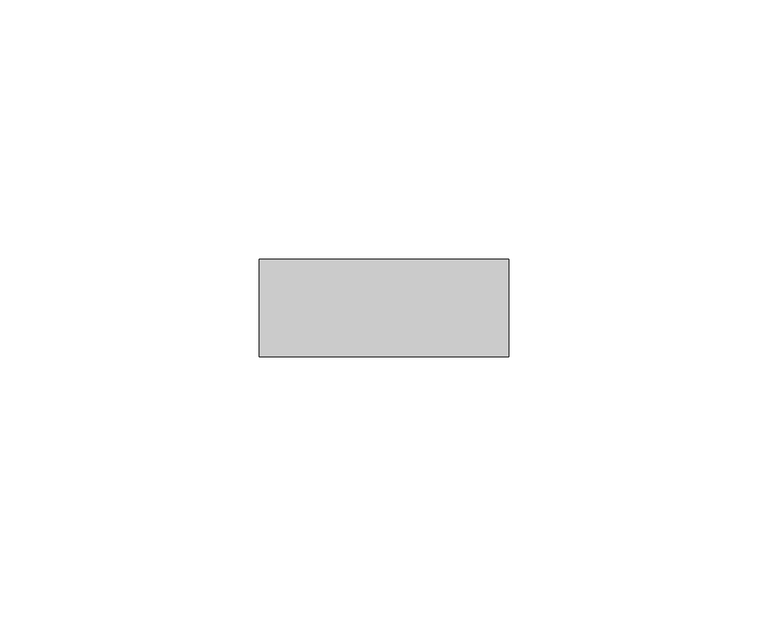
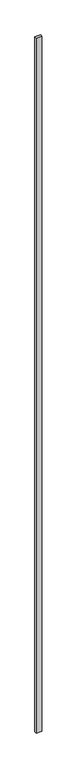
"""IFC4 building model written with IfcOpenShell, lengths in millimetres: proxy geometry, Generic Models 11:Generic Models 1:306267:Generic Models 1:306267 : Generic Models 11:Generic Models 1:306267:300405:Generic Models 1:306267:Generic Models 1:306267 : Generic Models 11:Generic Models 1:306267:300405 : Generic Models 11:Generic Models 1:306267:Generic Models 1:306267 : Generic Models 11:Generic Models 1:306267:300405:29 : Generic Models 11:Generic Models 1:306267:Generic Models 1:306267 : Generic Models 11:Generic Models 1:306267:300405:Generic Models 1:306267:Generic Models 1:306267 : Generic Models 11:Generic Models 1:306267:300405 : Generic Models 11:Generic Models 1:306267:Generic Models 1:306267 : Generic Models 11:Generic Models 1:306267:300405:300182."""

from ifc_helpers import new_model, si_unit, origin, origin_with_axes, place, context, project, spatial, polyline, outline, extrude, source, transform, mapped, element, save


def generic_models_2fd2b33c(model_context):
    return source(origin(), model_context, "Body", "SweptSolid", [
        extrude(outline(polyline([(667551.6493852, -568253.9540363), (667551.6493852, -568235.1560699), (667599.7284465, -568235.1560699), (667599.7284465, -568253.9540363), (667551.6493852, -568253.9540363)])), origin_with_axes(), (0.0, 0.0, 1.0), 6172.2),
    ])


if __name__ == "__main__":
    model = new_model("IFC4")
    model_context = context("Model", 3, world=origin())
    ifc_project = project(units=[si_unit("LENGTHUNIT", "METRE", prefix="MILLI")], contexts=[model_context])
    site = spatial("IfcSite", under=ifc_project)
    building = spatial("IfcBuilding", under=site)
    placement = place(None, origin())
    generic_models_shape = generic_models_2fd2b33c(model_context)
    element("IfcBuildingElementProxy", 1, Name="Generic Models 11:Generic Models 1:306267:Generic Models 1:306267 : Generic Models 11:Generic Models 1:306267:300405:Generic Models 1:306267:Generic Models 1:306267 : Generic Models 11:Generic Models 1:306267:300405 : Generic Models 11:Generic Models 1:306267:Generic Models 1:306267 : Generic Models 11:Generic Models 1:306267:300405:29 : Generic Models 11:Generic Models 1:306267:Generic Models 1:306267 : Generic Models 11:Generic Models 1:306267:300405:Generic Models 1:306267:Generic Models 1:306267 : Generic Models 11:Generic Models 1:306267:300405 : Generic Models 11:Generic Models 1:306267:Generic Models 1:306267 : Generic Models 11:Generic Models 1:306267:300405:300182", ObjectType="Generic Models 11:Generic Models 1:306267:Generic Models 1:306267 : Generic Models 11:Generic Models 1:306267:300405:Generic Models 1:306267:Generic Models 1:306267 : Generic Models 11:Generic Models 1:306267:300405 : Generic Models 11:Generic Models 1:306267:Generic Models 1:306267 : Generic Models 11:Generic Models 1:306267:300405:29 : Generic Models 11:Generic Models 1:306267:Generic Models 1:306267 : Generic Models 11:Generic Models 1:306267:300405:Generic Models 1:306267:Generic Models 1:306267 : Generic Models 11:Generic Models 1:306267:300405 : Generic Models 11:Generic Models 1:306267:Generic Models 1:306267 : Generic Models 11:Generic Models 1:306267:300405:300182", at=placement, inside=building, context=model_context, shape_type="MappedRepresentation", body=[
        mapped(generic_models_shape, transform((0.0, 0.0, 0.0), x_axis=(1.0, 0.0, 0.0), y_axis=(0.0, 1.0, 0.0), z_axis=(0.0, 0.0, 1.0))),
    ])
    save(model, "model.ifc")

# Revit data of these elements
# Type "Generic Models 11:Generic Models 1:306267:Generic Models 1:306267 : Generic Models 11:Generic Models 1:306267:300405:Generic Models 1:306267:Generic Models 1:306267 : Generic Models 11:Generic Models 1:306267:300405 : Generic Models 11:Generic Models 1:306267:Generic Models 1:306267 : Generic Models 11:Generic Models 1:306267:300405:29 : Generic Models 11:Generic Models 1:306267:Generic Models 1:306267 : Generic Models 11:Generic Models 1:306267:300405:Generic Models 1:306267:Generic Models 1:306267 : Generic Models 11:Generic Models 1:306267:300405 : Generic Models 11:Generic Models 1:306267:Generic Models 1:306267 : Generic Models 11:Generic Models 1:306267:300405:300182"
#   NameOverride = "Generic Models 11:Generic Models 1:306267:Generic Models 1:306267 : Generic Models 11:Generic Models 1:306267:300405:Generic Models 1:306267:Generic Models 1:306267 : Generic Models 11:Generic Models 1:306267:300405 : Generic Models 11:Generic Models 1:306267:Generic Models 1:306267 : Generic Models 11:Generic Models 1:306267:300405:300182"
#   ObjectTypeOverride = "Generic Models 1:306267:Generic Models 1:306267 : Generic Models 11:Generic Models 1:306267:300405 : Generic Models 11:Generic Models 1:306267:Generic Models 1:306267 : Generic Models 11:Generic Models 1:306267:300405"
#   Reference = "Generic Models 1"
#   Tag = "300182"
# Element 1 (IfcBuildingElementProxy, "Generic Models 11:Generic Models 1:306267:Generic Models 1:306267 : Generic Models 11:Generic Models 1:306267:300405:Generic Models 1:306267:Generic Models 1:306267 : Generic Models 11:Generic Models 1:306267:300405 : Generic Models 11:Generic Models 1:306267:Generic Models 1:306267 : Generic Models 11:Generic Models 1:306267:300405:29 : Generic Models 11:Generic Models 1:306267:Generic Models 1:306267 : Generic Models 11:Generic Models 1:306267:300405:Generic Models 1:306267:Generic Models 1:306267 : Generic Models 11:Generic Models 1:306267:300405 : Generic Models 11:Generic Models 1:306267:Generic Models 1:306267 : Generic Models 11:Generic Models 1:306267:300405:300182")
#   Materials on its faces: "WOOD BLOCKING - SIZE AS NECESSARY"
# Materials
#   "WOOD BLOCKING - SIZE AS NECESSARY": class "Wood", colour RGB 144 113 62, transparency 0, Description = "Pinus Echinata", Cost = 0
